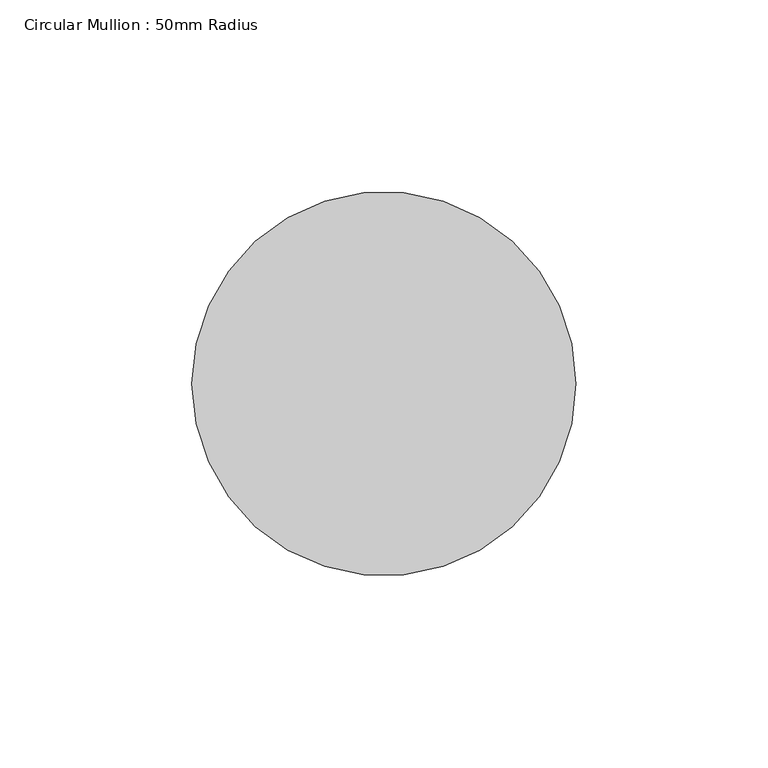
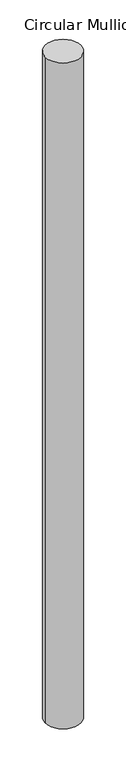
"""IFC4 building model written with IfcOpenShell, lengths in millimetres: member geometry, Circular Mullion : 50mm Radius."""

import ifcopenshell
import ifcopenshell.guid

model = None  # the IFC model being written
_history = None  # IfcOwnerHistory: only IFC2X3 demands one
_inside = {}  # id of a spatial element -> (the spatial element, [elements in it])
_under = {}  # id of a project, library or spatial element -> (it, [spatial elements below it])
_declared = {}  # id of a project -> (the project, [libraries it declares])
_typed = {}  # id of a type object -> (the type object, [elements of that type])
_made_of = {}  # id of a material, layer set ... -> (it, [elements and type objects made of it])


def new_model(schema):
    """Start an empty IFC model of exactly this schema.

    Asked for "IFC4X3", IfcOpenShell would pick the latest addendum, in which some entities
    have other attributes; the version numbers below select the first issue.
    IFC2X3 requires an IfcOwnerHistory on every rooted entity: one is made here for all.
    """
    global model, _history
    if schema == "IFC4X3":
        model = ifcopenshell.file(schema_version=(4, 3, 0, 0))
    else:
        model = ifcopenshell.file(schema=schema)
    _inside.clear()
    _under.clear()
    _declared.clear()
    _typed.clear()
    _made_of.clear()
    _history = None
    if model.schema == "IFC2X3":
        org = make("IfcOrganization", Name="unknown")
        user = make(
            "IfcPersonAndOrganization",
            ThePerson=make("IfcPerson", FamilyName="unknown"),
            TheOrganization=org,
        )
        app = make(
            "IfcApplication",
            ApplicationDeveloper=org,
            Version="unknown",
            ApplicationFullName="unknown",
            ApplicationIdentifier="unknown",
        )
        _history = make(
            "IfcOwnerHistory",
            OwningUser=user,
            OwningApplication=app,
            ChangeAction="ADDED",
            CreationDate=0,
        )
    return model


def make(cls, **values):
    """One entity of the class cls with the attributes given. An attribute that is None is left unset."""
    return model.create_entity(
        cls, **{name: value for name, value in values.items() if value is not None}
    )


def rooted(cls, **values):
    """An entity with a GlobalId (a new one), such as an element, a storey or a relation."""
    return make(cls, GlobalId=ifcopenshell.guid.new(), OwnerHistory=_history, **values)


def si_unit(unit_type, name, prefix=None):
    """IfcSIUnit, for example si_unit("LENGTHUNIT", "METRE", prefix="MILLI")."""
    return make("IfcSIUnit", UnitType=unit_type, Prefix=prefix, Name=name)


def assignment(units):
    """IfcUnitAssignment: the units of a project."""
    return None if units is None else make("IfcUnitAssignment", Units=units)


def point(xyz):
    """IfcCartesianPoint."""
    return None if xyz is None else make("IfcCartesianPoint", Coordinates=xyz)


def direction(xyz):
    """IfcDirection."""
    return None if xyz is None else make("IfcDirection", DirectionRatios=xyz)


def frame(location, z_axis=None, x_axis=None):
    """IfcAxis2Placement3D, a coordinate frame: its origin and axes. An axis left out is left unset."""
    return make(
        "IfcAxis2Placement3D",
        Location=point(location),
        Axis=direction(z_axis),
        RefDirection=direction(x_axis),
    )


def frame_2d(location, x_axis=None):
    """IfcAxis2Placement2D, a coordinate frame in the plane: its origin and x axis."""
    return make(
        "IfcAxis2Placement2D", Location=point(location), RefDirection=direction(x_axis)
    )


def origin():
    """The frame at (0, 0, 0) with its axes left unset."""
    return frame((0.0, 0.0, 0.0))


def place(relative_to, where):
    """IfcLocalPlacement: puts the frame where relative to a parent placement (None: the world)."""
    return make(
        "IfcLocalPlacement", PlacementRelTo=relative_to, RelativePlacement=where
    )


def context(
    kind, dimensions, precision=None, world=None, true_north=None, identifier=None
):
    """IfcGeometricRepresentationContext, for example the 3D "Model" context."""
    return make(
        "IfcGeometricRepresentationContext",
        ContextIdentifier=identifier,
        ContextType=kind,
        CoordinateSpaceDimension=dimensions,
        Precision=precision,
        WorldCoordinateSystem=world,
        TrueNorth=true_north,
    )


def project(units=None, contexts=None):
    """IfcProject with its units and contexts."""
    return rooted(
        "IfcProject",
        Name="project",
        RepresentationContexts=contexts,
        UnitsInContext=assignment(units),
    )


def spatial(cls, under=None, at=None, **own):
    """A site, building, storey or space (cls), placed at a placement, below another one or the project."""
    s = rooted(cls, ObjectPlacement=at, **own)
    if under is not None:
        _under.setdefault(under.id(), (under, []))[1].append(s)
    return s


def circle_curve(where, radius):
    """IfcCircle in the frame where."""
    return make("IfcCircle", Position=where, Radius=radius)


def trimmed(basis, trim1, trim2, sense, master):
    """IfcTrimmedCurve: the piece of a basis curve between two trims."""
    return make(
        "IfcTrimmedCurve",
        BasisCurve=basis,
        Trim1=trim1,
        Trim2=trim2,
        SenseAgreement=sense,
        MasterRepresentation=master,
    )


def segment(curve, same_sense, transition):
    """IfcCompositeCurveSegment."""
    return make(
        "IfcCompositeCurveSegment",
        Transition=transition,
        SameSense=same_sense,
        ParentCurve=curve,
    )


def composite_curve(segments, self_intersect=None):
    """IfcCompositeCurve: segments joined end to end."""
    return make("IfcCompositeCurve", Segments=segments, SelfIntersect=self_intersect)


def outline(outer, holes=None, kind="AREA"):
    """IfcArbitraryClosedProfileDef: a profile drawn as a closed curve; with holes, ...WithVoids."""
    if holes is None:
        return make("IfcArbitraryClosedProfileDef", ProfileType=kind, OuterCurve=outer)
    return make(
        "IfcArbitraryProfileDefWithVoids",
        ProfileType=kind,
        OuterCurve=outer,
        InnerCurves=holes,
    )


def extrude(swept, where, along, depth):
    """IfcExtrudedAreaSolid: the profile swept, set in the frame where, extruded along a direction by depth."""
    return make(
        "IfcExtrudedAreaSolid",
        SweptArea=swept,
        Position=where,
        ExtrudedDirection=direction(along),
        Depth=depth,
    )


def shape(context_of_items, identifier, shape_type, items):
    """IfcShapeRepresentation: the items that make up one representation, for example the "Body"."""
    return make(
        "IfcShapeRepresentation",
        ContextOfItems=context_of_items,
        RepresentationIdentifier=identifier,
        RepresentationType=shape_type,
        Items=items,
    )


def source(mapping_origin, context_of_items, identifier, shape_type, items):
    """IfcRepresentationMap: a shape defined once, which mapped items show again and again."""
    return make(
        "IfcRepresentationMap",
        MappingOrigin=mapping_origin,
        MappedRepresentation=shape(context_of_items, identifier, shape_type, items),
    )


def transform(
    local_origin,
    x_axis=None,
    y_axis=None,
    z_axis=None,
    scale=None,
    scale2=None,
    scale3=None,
    uniform=True,
):
    """IfcCartesianTransformationOperator3D, or its non-uniform kind. x_axis, y_axis, z_axis: its Axis1, 2, 3."""
    if uniform:
        return make(
            "IfcCartesianTransformationOperator3D",
            Axis1=direction(x_axis),
            Axis2=direction(y_axis),
            LocalOrigin=point(local_origin),
            Scale=scale,
            Axis3=direction(z_axis),
        )
    return make(
        "IfcCartesianTransformationOperator3DnonUniform",
        Axis1=direction(x_axis),
        Axis2=direction(y_axis),
        LocalOrigin=point(local_origin),
        Scale=scale,
        Axis3=direction(z_axis),
        Scale2=scale2,
        Scale3=scale3,
    )


def mapped(mapping_source, mapping_target):
    """IfcMappedItem: shows the shape of a source again, moved by a transform."""
    return make(
        "IfcMappedItem", MappingSource=mapping_source, MappingTarget=mapping_target
    )


def made_of(thing, what):
    """Note that an element or type object is made of a material, layer set ...; save() writes the relation."""
    if what is not None:
        _made_of.setdefault(what.id(), (what, []))[1].append(thing)
    return thing


def element(
    cls,
    number,
    at=None,
    inside=None,
    cuts=None,
    type_object=None,
    material=None,
    context=None,
    identifier="Body",
    shape_type=None,
    held_by="IfcProductDefinitionShape",
    body=None,
    shapes=None,
    **own,
):
    """One element of the class cls, such as IfcWall. Its Tag is "e" and its number.

    at: its placement. inside: the storey or other place that contains it. cuts: it is an
    opening in that element (IfcRelVoidsElement). A single representation is given by context,
    identifier, shape_type and body (its items); several are given by shapes. held_by: the class
    of the entity that holds the representations. save() writes the other relations.
    """
    e = rooted(cls, Tag="e%d" % number, ObjectPlacement=at, **own)
    if body is not None:
        shapes = [shape(context, identifier, shape_type, body)]
    if shapes is not None:
        e.Representation = make(held_by, Representations=shapes)
    if inside is not None:
        _inside.setdefault(inside.id(), (inside, []))[1].append(e)
    if cuts is not None:
        rooted(
            "IfcRelVoidsElement", RelatingBuildingElement=cuts, RelatedOpeningElement=e
        )
    if type_object is not None:
        _typed.setdefault(type_object.id(), (type_object, []))[1].append(e)
    return made_of(e, material)


def aggregate(whole, parts):
    """IfcRelAggregates: a whole, such as a stair, and the parts it consists of."""
    return rooted("IfcRelAggregates", RelatingObject=whole, RelatedObjects=parts)


def save(model, path):
    """Write the relations noted so far, then the file.

    IfcRelAggregates (storeys below a building ...), IfcRelContainedInSpatialStructure (elements
    in a storey), IfcRelDefinesByType, IfcRelAssociatesMaterial and IfcRelDeclares: one each for
    every whole, place, type object, material and project.
    """
    for whole, parts in _under.values():
        aggregate(whole, parts)
    for where, things in _inside.values():
        rooted(
            "IfcRelContainedInSpatialStructure",
            RelatedElements=things,
            RelatingStructure=where,
        )
    for kind, things in _typed.values():
        rooted("IfcRelDefinesByType", RelatedObjects=things, RelatingType=kind)
    for what, things in _made_of.values():
        rooted("IfcRelAssociatesMaterial", RelatedObjects=things, RelatingMaterial=what)
    for by, libraries in _declared.values():
        rooted("IfcRelDeclares", RelatingContext=by, RelatedDefinitions=libraries)
    model.write(path)


def circular_mullion_50mm_radius_814fe026(model_context):
    return source(origin(), model_context, "Body", "SweptSolid", [
        extrude(outline(composite_curve([segment(trimmed(circle_curve(frame_2d((-50.0, 0.0)), 50.0), [point((0.0, 0.0))], [point((-100.0, 0.0))], False, "CARTESIAN"), True, "CONTINUOUS"), segment(trimmed(circle_curve(frame_2d((-50.0, 0.0)), 50.0), [point((-100.0, 0.0))], [point((0.0, 0.0))], False, "CARTESIAN"), True, "CONTINUOUS")], self_intersect=False)), frame((0.0, 0.0, -1961.5145775), z_axis=(0.0, 0.0, 1.0), x_axis=(1.0, 0.0, 0.0)), (0.0, 0.0, 1.0), 1961.5145775),
    ])


if __name__ == "__main__":
    model = new_model("IFC4")
    model_context = context("Model", 3, world=origin())
    ifc_project = project(units=[si_unit("LENGTHUNIT", "METRE", prefix="MILLI")], contexts=[model_context])
    site = spatial("IfcSite", under=ifc_project)
    building = spatial("IfcBuilding", under=site)
    placement = place(None, origin())
    circular_mullion_50mm_radius_shape = circular_mullion_50mm_radius_814fe026(model_context)
    element("IfcMember", 1, ObjectType="Circular Mullion : 50mm Radius", at=placement, inside=building, context=model_context, shape_type="MappedRepresentation", body=[
        mapped(circular_mullion_50mm_radius_shape, transform((0.0, 0.0, 0.0), x_axis=(1.0, 0.0, 0.0), y_axis=(0.0, 1.0, 0.0), z_axis=(0.0, 0.0, 1.0))),
    ])
    save(model, "model.ifc")

# Revit data of these elements
# Type "Circular Mullion : 50mm Radius"
#   built-in parameter 1007350 = 0.164042 (stored number, unit not read)
# Element 1 (IfcMember, "Circular Mullion : 50mm Radius")
#   Materials on its faces: "Aluminium"
# Materials
#   "Aluminium": class "Metal", colour RGB 247 247 247, transparency 0, Description = "Aluminium 6061", Cost = 0
